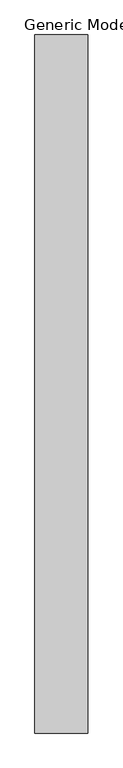
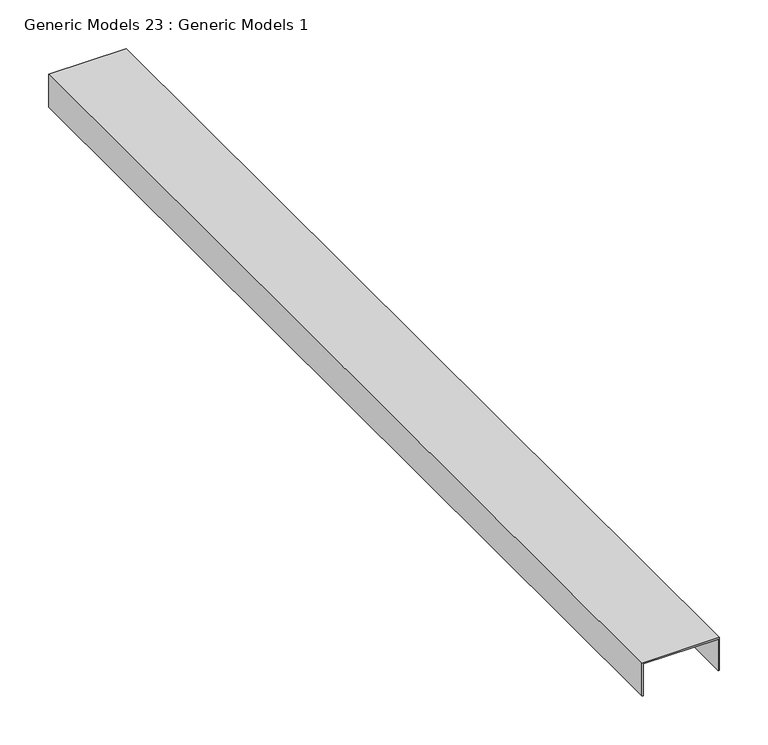
"""IFC4 building model written with IfcOpenShell, lengths in millimetres: proxy geometry, Generic Models 23 : Generic Models 1."""

from ifc_helpers import new_model, si_unit, frame, origin, place, context, project, spatial, polyline, outline, extrude, source, transform, mapped, element, save


def generic_models_23_generic_models_1_d2f1e0fb(model_context):
    return source(origin(), model_context, "Body", "SweptSolid", [
        extrude(outline(polyline([(2457.45, 49784.0), (2457.45, 49691.925), (2416.175, 49691.925), (2416.175, 49693.5125), (2455.8625, 49693.5125), (2455.8625, 49782.4125), (2416.175, 49782.4125), (2416.175, 49784.0), (2457.45, 49784.0)])), frame((0.0, 0.0, 0.0), z_axis=(0.0, 1.0, 0.0), x_axis=(0.0, 0.0, 1.0)), (0.0, 0.0, 1.0), 1219.2),
    ])


if __name__ == "__main__":
    model = new_model("IFC4")
    model_context = context("Model", 3, world=origin())
    ifc_project = project(units=[si_unit("LENGTHUNIT", "METRE", prefix="MILLI")], contexts=[model_context])
    site = spatial("IfcSite", under=ifc_project)
    building = spatial("IfcBuilding", under=site)
    placement = place(None, origin())
    generic_models_23_generic_models_1_shape = generic_models_23_generic_models_1_d2f1e0fb(model_context)
    element("IfcBuildingElementProxy", 1, Name="Generic Models 23 : Generic Models 1", ObjectType="Generic Models 23 : Generic Models 1", at=placement, inside=building, context=model_context, shape_type="MappedRepresentation", body=[
        mapped(generic_models_23_generic_models_1_shape, transform((0.0, 0.0, 0.0), x_axis=(1.0, 0.0, 0.0), y_axis=(0.0, 1.0, 0.0), z_axis=(0.0, 0.0, 1.0))),
    ])
    save(model, "model.ifc")

# Revit data of these elements
# Element 1 (IfcBuildingElementProxy, "Generic Models 23 : Generic Models 1")
#   Materials on its faces: "MATCH DEPTH OF EXISTING DEFLECTION TRACK"
# Materials
#   "MATCH DEPTH OF EXISTING DEFLECTION TRACK": class "Unassigned", colour RGB 210 209 208, transparency 0, Keynote = "M05121300.02", Cost = 0
